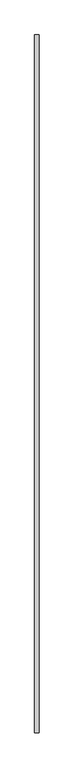
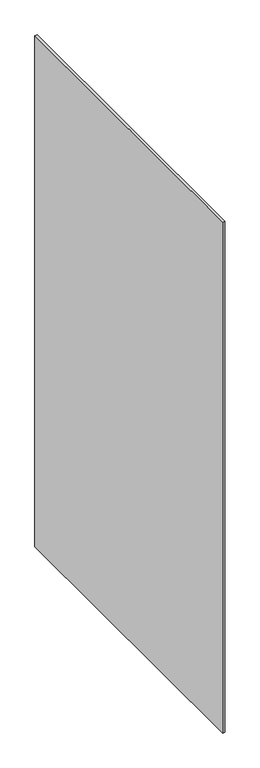
"""IFC4 building model written with IfcOpenShell, lengths in millimetres: proxy geometry, Panel:Panel:300402:Panel:300402 : Panel:Panel:300402:300124:Panel:300402:Panel:300402 : Panel:Panel:300402:300124 : Panel:Panel:300402:Panel:300402 : Panel:Panel:300402:300124:9 : Panel:Panel:300402:Panel:300402 : Panel:Panel:300402:300124:Panel:300402:Panel:300402 : Panel:Panel:300402:300124 : Panel:Panel:300402:Panel:300402 : Panel:Panel:300402:300124:300083."""

from ifc_helpers import new_model, si_unit, frame, origin, place, context, project, spatial, polyline, outline, extrude, source, transform, mapped, element, save


def generic_models_0687ebd7(model_context):
    return source(origin(), model_context, "Body", "SweptSolid", [
        extrude(outline(polyline([(579383.9117239, -577498.9163841), (579391.8492239, -577498.9163841), (579391.8492239, -578718.1163841), (579383.9117239, -578718.1163841), (579383.9117239, -577498.9163841)])), frame((0.0, 0.0, 4107.2166439), z_axis=(0.0, 0.0, 1.0), x_axis=(1.0, 0.0, 0.0)), (0.0, 0.0, 1.0), 2026.8833561),
    ])


if __name__ == "__main__":
    model = new_model("IFC4")
    model_context = context("Model", 3, world=origin())
    ifc_project = project(units=[si_unit("LENGTHUNIT", "METRE", prefix="MILLI")], contexts=[model_context])
    site = spatial("IfcSite", under=ifc_project)
    building = spatial("IfcBuilding", under=site)
    placement = place(None, origin())
    generic_models_shape = generic_models_0687ebd7(model_context)
    element("IfcBuildingElementProxy", 1, Name="Panel:Panel:300402:Panel:300402 : Panel:Panel:300402:300124:Panel:300402:Panel:300402 : Panel:Panel:300402:300124 : Panel:Panel:300402:Panel:300402 : Panel:Panel:300402:300124:9 : Panel:Panel:300402:Panel:300402 : Panel:Panel:300402:300124:Panel:300402:Panel:300402 : Panel:Panel:300402:300124 : Panel:Panel:300402:Panel:300402 : Panel:Panel:300402:300124:300083", ObjectType="Panel:Panel:300402:Panel:300402 : Panel:Panel:300402:300124:Panel:300402:Panel:300402 : Panel:Panel:300402:300124 : Panel:Panel:300402:Panel:300402 : Panel:Panel:300402:300124:9 : Panel:Panel:300402:Panel:300402 : Panel:Panel:300402:300124:Panel:300402:Panel:300402 : Panel:Panel:300402:300124 : Panel:Panel:300402:Panel:300402 : Panel:Panel:300402:300124:300083", at=placement, inside=building, context=model_context, shape_type="MappedRepresentation", body=[
        mapped(generic_models_shape, transform((0.0, 0.0, 0.0), x_axis=(1.0, 0.0, 0.0), y_axis=(0.0, 1.0, 0.0), z_axis=(0.0, 0.0, 1.0))),
    ])
    save(model, "model.ifc")

# Revit data of these elements
# Type "Panel:Panel:300402:Panel:300402 : Panel:Panel:300402:300124:Panel:300402:Panel:300402 : Panel:Panel:300402:300124 : Panel:Panel:300402:Panel:300402 : Panel:Panel:300402:300124:9 : Panel:Panel:300402:Panel:300402 : Panel:Panel:300402:300124:Panel:300402:Panel:300402 : Panel:Panel:300402:300124 : Panel:Panel:300402:Panel:300402 : Panel:Panel:300402:300124:300083"
#   NameOverride = "Panel:Panel:300402:Panel:300402 : Panel:Panel:300402:300124:Panel:300402:Panel:300402 : Panel:Panel:300402:300124 : Panel:Panel:300402:Panel:300402 : Panel:Panel:300402:300124:300083"
#   ObjectTypeOverride = "Panel:300402:Panel:300402 : Panel:Panel:300402:300124 : Panel:Panel:300402:Panel:300402 : Panel:Panel:300402:300124"
#   Reference = "Panel"
#   Tag = "300083"
# Element 1 (IfcBuildingElementProxy, "Panel:Panel:300402:Panel:300402 : Panel:Panel:300402:300124:Panel:300402:Panel:300402 : Panel:Panel:300402:300124 : Panel:Panel:300402:Panel:300402 : Panel:Panel:300402:300124:9 : Panel:Panel:300402:Panel:300402 : Panel:Panel:300402:300124:Panel:300402:Panel:300402 : Panel:Panel:300402:300124 : Panel:Panel:300402:Panel:300402 : Panel:Panel:300402:300124:300083")
#   Materials on its faces: "5/16\" THICK STONEWOOD RESIN PANELS - EXPOSED FASTENERS"
# Materials
#   "5/16\" THICK STONEWOOD RESIN PANELS - EXPOSED FASTENERS": class "Unassigned", colour RGB 64 64 64, transparency 0, Keynote = "M07420000.01", Cost = 0
